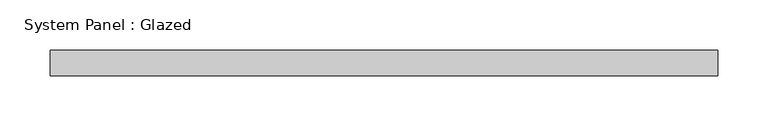
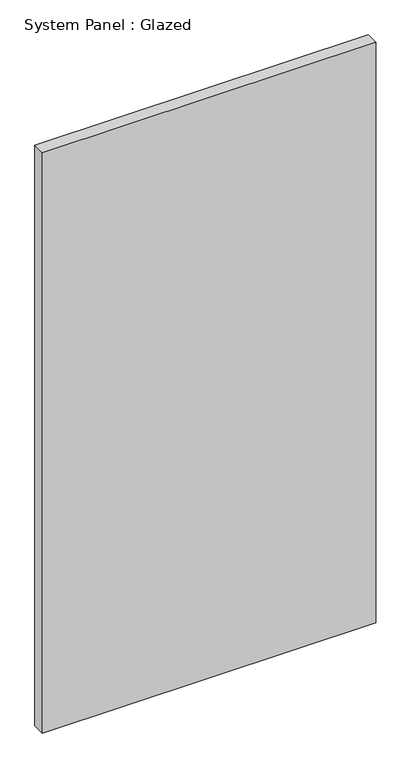
"""IFC4 building model written with IfcOpenShell, lengths in millimetres: plate geometry, System Panel : Glazed."""

import ifcopenshell
import ifcopenshell.guid

model = None  # the IFC model being written
_history = None  # IfcOwnerHistory: only IFC2X3 demands one
_inside = {}  # id of a spatial element -> (the spatial element, [elements in it])
_under = {}  # id of a project, library or spatial element -> (it, [spatial elements below it])
_declared = {}  # id of a project -> (the project, [libraries it declares])
_typed = {}  # id of a type object -> (the type object, [elements of that type])
_made_of = {}  # id of a material, layer set ... -> (it, [elements and type objects made of it])


def new_model(schema):
    """Start an empty IFC model of exactly this schema.

    Asked for "IFC4X3", IfcOpenShell would pick the latest addendum, in which some entities
    have other attributes; the version numbers below select the first issue.
    IFC2X3 requires an IfcOwnerHistory on every rooted entity: one is made here for all.
    """
    global model, _history
    if schema == "IFC4X3":
        model = ifcopenshell.file(schema_version=(4, 3, 0, 0))
    else:
        model = ifcopenshell.file(schema=schema)
    _inside.clear()
    _under.clear()
    _declared.clear()
    _typed.clear()
    _made_of.clear()
    _history = None
    if model.schema == "IFC2X3":
        org = make("IfcOrganization", Name="unknown")
        user = make(
            "IfcPersonAndOrganization",
            ThePerson=make("IfcPerson", FamilyName="unknown"),
            TheOrganization=org,
        )
        app = make(
            "IfcApplication",
            ApplicationDeveloper=org,
            Version="unknown",
            ApplicationFullName="unknown",
            ApplicationIdentifier="unknown",
        )
        _history = make(
            "IfcOwnerHistory",
            OwningUser=user,
            OwningApplication=app,
            ChangeAction="ADDED",
            CreationDate=0,
        )
    return model


def make(cls, **values):
    """One entity of the class cls with the attributes given. An attribute that is None is left unset."""
    return model.create_entity(
        cls, **{name: value for name, value in values.items() if value is not None}
    )


def rooted(cls, **values):
    """An entity with a GlobalId (a new one), such as an element, a storey or a relation."""
    return make(cls, GlobalId=ifcopenshell.guid.new(), OwnerHistory=_history, **values)


def si_unit(unit_type, name, prefix=None):
    """IfcSIUnit, for example si_unit("LENGTHUNIT", "METRE", prefix="MILLI")."""
    return make("IfcSIUnit", UnitType=unit_type, Prefix=prefix, Name=name)


def assignment(units):
    """IfcUnitAssignment: the units of a project."""
    return None if units is None else make("IfcUnitAssignment", Units=units)


def point(xyz):
    """IfcCartesianPoint."""
    return None if xyz is None else make("IfcCartesianPoint", Coordinates=xyz)


def direction(xyz):
    """IfcDirection."""
    return None if xyz is None else make("IfcDirection", DirectionRatios=xyz)


def frame(location, z_axis=None, x_axis=None):
    """IfcAxis2Placement3D, a coordinate frame: its origin and axes. An axis left out is left unset."""
    return make(
        "IfcAxis2Placement3D",
        Location=point(location),
        Axis=direction(z_axis),
        RefDirection=direction(x_axis),
    )


def origin():
    """The frame at (0, 0, 0) with its axes left unset."""
    return frame((0.0, 0.0, 0.0))


def origin_with_axes():
    """The frame at (0, 0, 0) with the z axis (0, 0, 1) and the x axis (1, 0, 0) written out."""
    return frame((0.0, 0.0, 0.0), z_axis=(0.0, 0.0, 1.0), x_axis=(1.0, 0.0, 0.0))


def place(relative_to, where):
    """IfcLocalPlacement: puts the frame where relative to a parent placement (None: the world)."""
    return make(
        "IfcLocalPlacement", PlacementRelTo=relative_to, RelativePlacement=where
    )


def context(
    kind, dimensions, precision=None, world=None, true_north=None, identifier=None
):
    """IfcGeometricRepresentationContext, for example the 3D "Model" context."""
    return make(
        "IfcGeometricRepresentationContext",
        ContextIdentifier=identifier,
        ContextType=kind,
        CoordinateSpaceDimension=dimensions,
        Precision=precision,
        WorldCoordinateSystem=world,
        TrueNorth=true_north,
    )


def project(units=None, contexts=None):
    """IfcProject with its units and contexts."""
    return rooted(
        "IfcProject",
        Name="project",
        RepresentationContexts=contexts,
        UnitsInContext=assignment(units),
    )


def spatial(cls, under=None, at=None, **own):
    """A site, building, storey or space (cls), placed at a placement, below another one or the project."""
    s = rooted(cls, ObjectPlacement=at, **own)
    if under is not None:
        _under.setdefault(under.id(), (under, []))[1].append(s)
    return s


def polyline(points):
    """IfcPolyline through the points."""
    return make("IfcPolyline", Points=[point(p) for p in points])


def outline(outer, holes=None, kind="AREA"):
    """IfcArbitraryClosedProfileDef: a profile drawn as a closed curve; with holes, ...WithVoids."""
    if holes is None:
        return make("IfcArbitraryClosedProfileDef", ProfileType=kind, OuterCurve=outer)
    return make(
        "IfcArbitraryProfileDefWithVoids",
        ProfileType=kind,
        OuterCurve=outer,
        InnerCurves=holes,
    )


def extrude(swept, where, along, depth):
    """IfcExtrudedAreaSolid: the profile swept, set in the frame where, extruded along a direction by depth."""
    return make(
        "IfcExtrudedAreaSolid",
        SweptArea=swept,
        Position=where,
        ExtrudedDirection=direction(along),
        Depth=depth,
    )


def shape(context_of_items, identifier, shape_type, items):
    """IfcShapeRepresentation: the items that make up one representation, for example the "Body"."""
    return make(
        "IfcShapeRepresentation",
        ContextOfItems=context_of_items,
        RepresentationIdentifier=identifier,
        RepresentationType=shape_type,
        Items=items,
    )


def source(mapping_origin, context_of_items, identifier, shape_type, items):
    """IfcRepresentationMap: a shape defined once, which mapped items show again and again."""
    return make(
        "IfcRepresentationMap",
        MappingOrigin=mapping_origin,
        MappedRepresentation=shape(context_of_items, identifier, shape_type, items),
    )


def transform(
    local_origin,
    x_axis=None,
    y_axis=None,
    z_axis=None,
    scale=None,
    scale2=None,
    scale3=None,
    uniform=True,
):
    """IfcCartesianTransformationOperator3D, or its non-uniform kind. x_axis, y_axis, z_axis: its Axis1, 2, 3."""
    if uniform:
        return make(
            "IfcCartesianTransformationOperator3D",
            Axis1=direction(x_axis),
            Axis2=direction(y_axis),
            LocalOrigin=point(local_origin),
            Scale=scale,
            Axis3=direction(z_axis),
        )
    return make(
        "IfcCartesianTransformationOperator3DnonUniform",
        Axis1=direction(x_axis),
        Axis2=direction(y_axis),
        LocalOrigin=point(local_origin),
        Scale=scale,
        Axis3=direction(z_axis),
        Scale2=scale2,
        Scale3=scale3,
    )


def mapped(mapping_source, mapping_target):
    """IfcMappedItem: shows the shape of a source again, moved by a transform."""
    return make(
        "IfcMappedItem", MappingSource=mapping_source, MappingTarget=mapping_target
    )


def made_of(thing, what):
    """Note that an element or type object is made of a material, layer set ...; save() writes the relation."""
    if what is not None:
        _made_of.setdefault(what.id(), (what, []))[1].append(thing)
    return thing


def element(
    cls,
    number,
    at=None,
    inside=None,
    cuts=None,
    type_object=None,
    material=None,
    context=None,
    identifier="Body",
    shape_type=None,
    held_by="IfcProductDefinitionShape",
    body=None,
    shapes=None,
    **own,
):
    """One element of the class cls, such as IfcWall. Its Tag is "e" and its number.

    at: its placement. inside: the storey or other place that contains it. cuts: it is an
    opening in that element (IfcRelVoidsElement). A single representation is given by context,
    identifier, shape_type and body (its items); several are given by shapes. held_by: the class
    of the entity that holds the representations. save() writes the other relations.
    """
    e = rooted(cls, Tag="e%d" % number, ObjectPlacement=at, **own)
    if body is not None:
        shapes = [shape(context, identifier, shape_type, body)]
    if shapes is not None:
        e.Representation = make(held_by, Representations=shapes)
    if inside is not None:
        _inside.setdefault(inside.id(), (inside, []))[1].append(e)
    if cuts is not None:
        rooted(
            "IfcRelVoidsElement", RelatingBuildingElement=cuts, RelatedOpeningElement=e
        )
    if type_object is not None:
        _typed.setdefault(type_object.id(), (type_object, []))[1].append(e)
    return made_of(e, material)


def aggregate(whole, parts):
    """IfcRelAggregates: a whole, such as a stair, and the parts it consists of."""
    return rooted("IfcRelAggregates", RelatingObject=whole, RelatedObjects=parts)


def save(model, path):
    """Write the relations noted so far, then the file.

    IfcRelAggregates (storeys below a building ...), IfcRelContainedInSpatialStructure (elements
    in a storey), IfcRelDefinesByType, IfcRelAssociatesMaterial and IfcRelDeclares: one each for
    every whole, place, type object, material and project.
    """
    for whole, parts in _under.values():
        aggregate(whole, parts)
    for where, things in _inside.values():
        rooted(
            "IfcRelContainedInSpatialStructure",
            RelatedElements=things,
            RelatingStructure=where,
        )
    for kind, things in _typed.values():
        rooted("IfcRelDefinesByType", RelatedObjects=things, RelatingType=kind)
    for what, things in _made_of.values():
        rooted("IfcRelAssociatesMaterial", RelatedObjects=things, RelatingMaterial=what)
    for by, libraries in _declared.values():
        rooted("IfcRelDeclares", RelatingContext=by, RelatedDefinitions=libraries)
    model.write(path)


def system_panel_glazed_f8e7f2c7(model_context):
    return source(origin(), model_context, "Body", "SweptSolid", [
        extrude(outline(polyline([(331.132211, 19.05), (-331.132211, 19.05), (-331.132211, 44.45), (331.132211, 44.45), (331.132211, 19.05)])), origin_with_axes(), (0.0, 0.0, 1.0), 1219.2),
    ])


if __name__ == "__main__":
    model = new_model("IFC4")
    model_context = context("Model", 3, world=origin())
    ifc_project = project(units=[si_unit("LENGTHUNIT", "METRE", prefix="MILLI")], contexts=[model_context])
    site = spatial("IfcSite", under=ifc_project)
    building = spatial("IfcBuilding", under=site)
    placement = place(None, origin())
    system_panel_glazed_shape = system_panel_glazed_f8e7f2c7(model_context)
    element("IfcPlate", 1, ObjectType="System Panel : Glazed", at=placement, inside=building, context=model_context, shape_type="MappedRepresentation", body=[
        mapped(system_panel_glazed_shape, transform((0.0, 0.0, 0.0), x_axis=(1.0, 0.0, 0.0), y_axis=(0.0, 1.0, 0.0), z_axis=(0.0, 0.0, 1.0))),
    ])
    save(model, "model.ifc")

# Revit data of these elements
# Element 1 (IfcPlate, "System Panel : Glazed")
#   Materials on its faces: "Glass"
# Materials
#   "Glass": class "Glass", colour RGB 0 128 192, transparency 0.75
